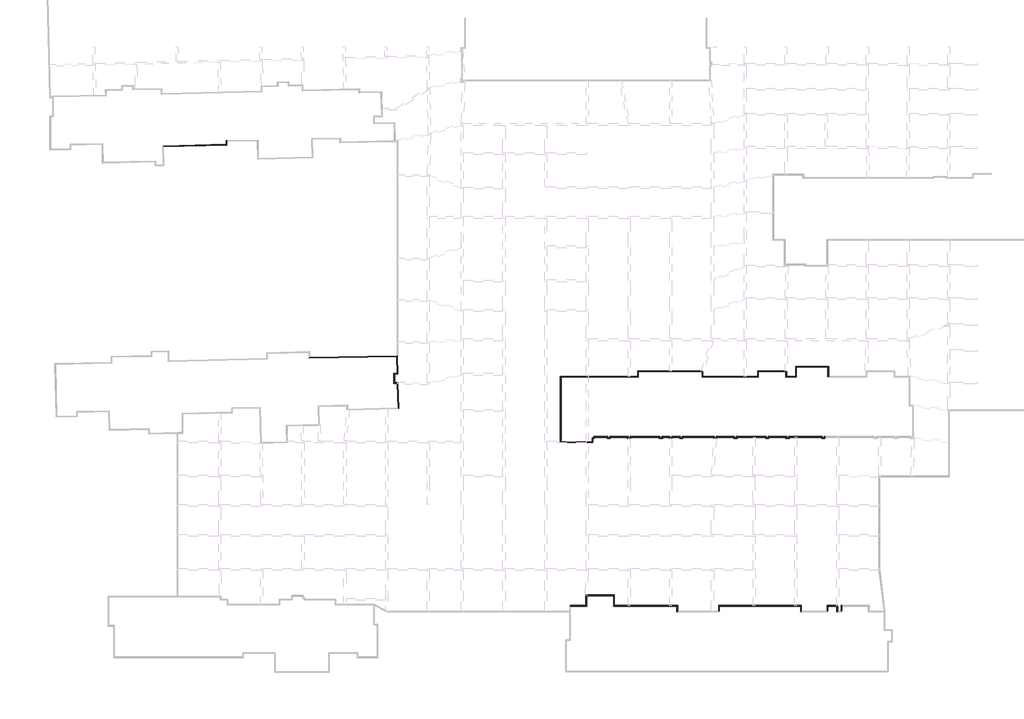
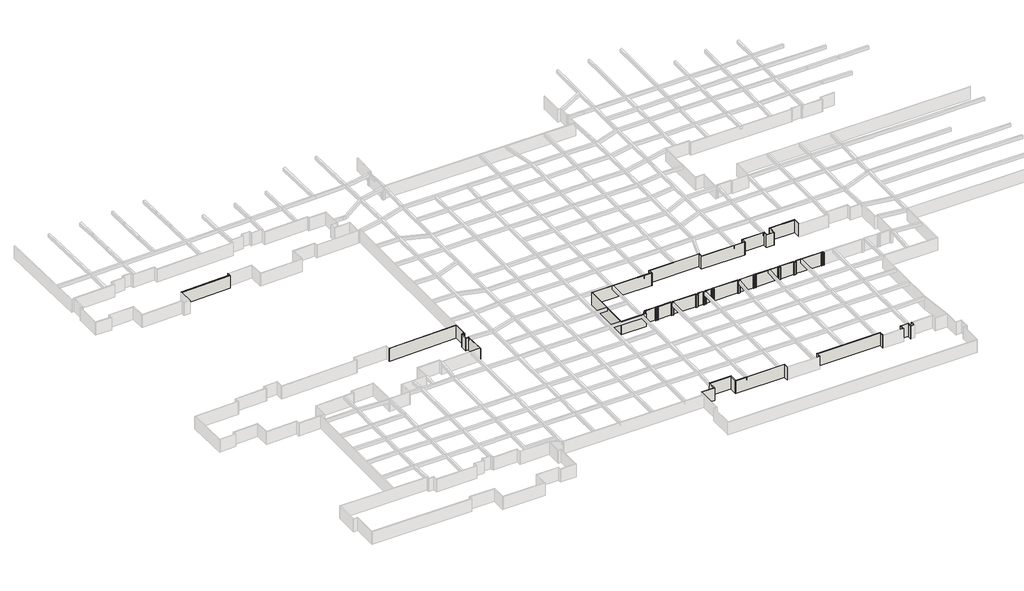
# One storey, part 3 of 20: 78 walls.
"""IFC4 building model written with IfcOpenShell, lengths in millimetres."""

from ifc_helpers import new_model, si_unit, origin, origin_with_axes, place, context, project, spatial, polyline, outline, extrude, faceted_brep, element, save

model = new_model("IFC4")

# Units and contexts
model_context = context("Model", 3, world=origin())
ifc_project = project(units=[si_unit("LENGTHUNIT", "METRE", prefix="MILLI")], contexts=[model_context])

# Site, building, storey
site = spatial("IfcSite", under=ifc_project)
building = spatial("IfcBuilding", under=site)
storey = spatial("IfcBuildingStorey", under=building, Name="户型图", Elevation=0.0)

# Walls
placement = place(None, origin())
element("IfcWall", 1, ObjectType="所有墙体", at=placement, inside=storey, context=model_context, shape_type="Brep", body=[
    faceted_brep([(-2724.8650084, 89257.8239839, 0.0), (9470.1632227, 89551.8005582, 0.0), (9470.1632227, 89551.8005582, 3300.0), (-2724.8650084, 89257.8239839, 3300.0), (-2727.75692, 89377.7891324, 0.0), (-2727.75692, 89377.7891324, 3300.0), (9350.1632227, 89668.9426681, 3300.0), (9470.1632227, 89671.8354198, 3300.0), (9470.1632227, 89671.8354198, 0.0), (9350.1632227, 89668.9426681, 0.0)], [[[0, 1, 2, 3]], [[4, 5, 6, 7, 8, 9]], [[1, 0, 4, 9, 8]], [[3, 2, 7, 6, 5]], [[0, 3, 5, 4]], [[2, 1, 8, 7]]]),
])
element("IfcWall", 2, ObjectType="所有墙体", at=placement, inside=storey, context=model_context, shape_type="Brep", body=[
    faceted_brep([(9470.1632227, 89671.8354198, 0.0), (9470.1632227, 90251.8005582, 0.0), (9470.1632227, 90371.8354198, 0.0), (9470.1632227, 90371.8354198, 3300.0), (9470.1632227, 90251.8005582, 3300.0), (9470.1632227, 89671.8354198, 3300.0), (9350.1632227, 89668.9426681, 0.0), (9350.1632227, 89668.9426681, 3300.0), (9350.1632227, 90368.9426681, 3300.0), (9350.1632227, 90368.9426681, 0.0)], [[[0, 1, 2, 3, 4, 5]], [[6, 7, 8, 9]], [[2, 1, 0, 6, 9]], [[5, 4, 3, 8, 7]], [[0, 5, 7, 6]], [[3, 2, 9, 8]]]),
])
element("IfcWall", 3, ObjectType="所有墙体", at=placement, inside=storey, context=model_context, shape_type="Brep", body=[
    faceted_brep([(42190.0, 49087.0906084, 0.0), (25412.5739519, 48794.2395474, 0.0), (25292.5739519, 48792.1449396, 0.0), (25292.5739519, 48792.1449396, 3300.0), (25412.5739519, 48794.2395474, 3300.0), (42190.0, 49087.0906084, 3300.0), (42190.0, 48967.072329, 0.0), (42190.0, 48967.072329, 3300.0), (42078.6480995, 48965.1286744, 3300.0), (25292.5739519, 48672.1266602, 3300.0), (25292.5739519, 48672.1266602, 0.0), (42078.6480995, 48965.1286744, 0.0)], [[[0, 1, 2, 3, 4, 5]], [[6, 7, 8, 9, 10, 11]], [[2, 1, 0, 6, 11, 10]], [[5, 4, 3, 9, 8, 7]], [[0, 5, 7, 6]], [[3, 2, 10, 9]]]),
])
element("IfcWall", 4, ObjectType="所有墙体", at=placement, inside=storey, context=model_context, shape_type="Brep", body=[
    faceted_brep([(75347.25326, 1046.0, 0.0), (78482.0, 1046.0, 0.0), (78482.0, 1046.0, 3300.0), (75347.25326, 1046.0, 3300.0), (75347.25326, 1166.0, 0.0), (75347.25326, 1166.0, 3300.0), (78362.0, 1166.0, 3300.0), (78482.0, 1166.0, 3300.0), (78482.0, 1166.0, 0.0), (78362.0, 1166.0, 0.0)], [[[0, 1, 2, 3]], [[4, 5, 6, 7, 8, 9]], [[1, 0, 4, 9, 8]], [[3, 2, 7, 6, 5]], [[0, 3, 5, 4]], [[2, 1, 8, 7]]]),
])
element("IfcWall", 5, ObjectType="所有墙体", at=placement, inside=storey, context=model_context, shape_type="Brep", body=[
    faceted_brep([(78482.0, 1166.0, 0.0), (78482.0, 3045.0, 0.0), (78482.0, 3165.0, 0.0), (78482.0, 3165.0, 3300.0), (78482.0, 3045.0, 3300.0), (78482.0, 1166.0, 3300.0), (78362.0, 1166.0, 0.0), (78362.0, 1166.0, 3300.0), (78362.0, 3165.0, 3300.0), (78362.0, 3165.0, 0.0)], [[[0, 1, 2, 3, 4, 5]], [[6, 7, 8, 9]], [[2, 1, 0, 6, 9]], [[5, 4, 3, 8, 7]], [[0, 5, 7, 6]], [[3, 2, 9, 8]]]),
])
element("IfcWall", 6, ObjectType="所有墙体", at=placement, inside=storey, context=model_context, shape_type="Brep", body=[
    faceted_brep([(78482.0, 3045.0, 0.0), (83662.0, 3045.0, 0.0), (83782.0, 3045.0, 0.0), (83782.0, 3045.0, 3300.0), (83662.0, 3045.0, 3300.0), (78482.0, 3045.0, 3300.0), (78482.0, 3165.0, 0.0), (78482.0, 3165.0, 3300.0), (83782.0, 3165.0, 3300.0), (83782.0, 3165.0, 0.0)], [[[0, 1, 2, 3, 4, 5]], [[6, 7, 8, 9]], [[2, 1, 0, 6, 9]], [[5, 4, 3, 8, 7]], [[0, 5, 7, 6]], [[3, 2, 9, 8]]]),
])
element("IfcWall", 7, ObjectType="所有墙体", at=placement, inside=storey, context=model_context, shape_type="Brep", body=[
    faceted_brep([(83662.0, 3045.0, 0.0), (83662.0, 1046.0, 0.0), (83662.0, 1046.0, 3300.0), (83662.0, 3045.0, 3300.0), (83782.0, 3045.0, 0.0), (83782.0, 3045.0, 3300.0), (83782.0, 1166.0, 3300.0), (83782.0, 1046.0, 3300.0), (83782.0, 1046.0, 0.0), (83782.0, 1166.0, 0.0)], [[[0, 1, 2, 3]], [[4, 5, 6, 7, 8, 9]], [[1, 0, 4, 9, 8]], [[3, 2, 7, 6, 5]], [[0, 3, 5, 4]], [[2, 1, 8, 7]]]),
])
element("IfcWall", 8, ObjectType="所有墙体", at=placement, inside=storey, context=model_context, shape_type="Brep", body=[
    faceted_brep([(83782.0, 1046.0, 0.0), (95812.0, 1046.0, 0.0), (95932.0, 1046.0, 0.0), (95932.0, 1046.0, 3300.0), (95812.0, 1046.0, 3300.0), (83782.0, 1046.0, 3300.0), (83782.0, 1166.0, 0.0), (83782.0, 1166.0, 3300.0), (95932.0, 1166.0, 3300.0), (95932.0, 1166.0, 0.0)], [[[0, 1, 2, 3, 4, 5]], [[6, 7, 8, 9]], [[2, 1, 0, 6, 9]], [[5, 4, 3, 8, 7]], [[0, 5, 7, 6]], [[3, 2, 9, 8]]]),
])
element("IfcWall", 9, ObjectType="所有墙体", at=placement, inside=storey, context=model_context, shape_type="Brep", body=[
    faceted_brep([(95812.0, 1046.0, 0.0), (95812.0, -63.5203758, 0.0), (95812.0, -63.5203758, 3300.0), (95812.0, 1046.0, 3300.0), (95932.0, 1046.0, 0.0), (95932.0, 1046.0, 3300.0), (95932.0, 56.4796242, 3300.0), (95932.0, -63.5203758, 3300.0), (95932.0, -63.5203758, 0.0), (95932.0, 56.4796242, 0.0)], [[[0, 1, 2, 3]], [[4, 5, 6, 7, 8, 9]], [[1, 0, 4, 9, 8]], [[3, 2, 7, 6, 5]], [[0, 3, 5, 4]], [[2, 1, 8, 7]]]),
])
element("IfcWall", 10, ObjectType="所有墙体", at=placement, inside=storey, context=model_context, shape_type="Brep", body=[
    faceted_brep([(103982.0, 56.4796242, 0.0), (103982.0, 1046.0, 0.0), (103982.0, 1166.0, 0.0), (103982.0, 1166.0, 3300.0), (103982.0, 1046.0, 3300.0), (103982.0, 56.4796242, 3300.0), (103862.0, 56.4796242, 0.0), (103862.0, 56.4796242, 3300.0), (103862.0, 1166.0, 3300.0), (103862.0, 1166.0, 0.0)], [[[0, 1, 2, 3, 4, 5]], [[6, 7, 8, 9]], [[2, 1, 0, 6, 9]], [[5, 4, 3, 8, 7]], [[0, 5, 7, 6]], [[3, 2, 9, 8]]]),
])
element("IfcWall", 11, ObjectType="所有墙体", at=placement, inside=storey, context=model_context, shape_type="Brep", body=[
    faceted_brep([(103982.0, 1046.0, 0.0), (119562.0, 1046.0, 0.0), (119682.0, 1046.0, 0.0), (119682.0, 1046.0, 3300.0), (119562.0, 1046.0, 3300.0), (103982.0, 1046.0, 3300.0), (103982.0, 1166.0, 0.0), (103982.0, 1166.0, 3300.0), (119682.0, 1166.0, 3300.0), (119682.0, 1166.0, 0.0)], [[[0, 1, 2, 3, 4, 5]], [[6, 7, 8, 9]], [[2, 1, 0, 6, 9]], [[5, 4, 3, 8, 7]], [[0, 5, 7, 6]], [[3, 2, 9, 8]]]),
])
element("IfcWall", 12, ObjectType="所有墙体", at=placement, inside=storey, context=model_context, shape_type="Brep", body=[
    faceted_brep([(119562.0, 1046.0, 0.0), (119562.0, -63.5203758, 0.0), (119562.0, -63.5203758, 3300.0), (119562.0, 1046.0, 3300.0), (119682.0, 1046.0, 0.0), (119682.0, 1046.0, 3300.0), (119682.0, 56.4796242, 3300.0), (119682.0, -63.5203758, 3300.0), (119682.0, -63.5203758, 0.0), (119682.0, 56.4796242, 0.0)], [[[0, 1, 2, 3]], [[4, 5, 6, 7, 8, 9]], [[1, 0, 4, 9, 8]], [[3, 2, 7, 6, 5]], [[0, 3, 5, 4]], [[2, 1, 8, 7]]]),
])
element("IfcWall", 13, ObjectType="所有墙体", at=placement, inside=storey, context=model_context, shape_type="Brep", body=[
    faceted_brep([(124732.0, 56.4796242, 0.0), (124732.0, 1046.0, 0.0), (124732.0, 1166.0, 0.0), (124732.0, 1166.0, 3300.0), (124732.0, 1046.0, 3300.0), (124732.0, 56.4796242, 3300.0), (124612.0, 56.4796242, 0.0), (124612.0, 56.4796242, 3300.0), (124612.0, 1166.0, 3300.0), (124612.0, 1166.0, 0.0)], [[[0, 1, 2, 3, 4, 5]], [[6, 7, 8, 9]], [[2, 1, 0, 6, 9]], [[5, 4, 3, 8, 7]], [[0, 5, 7, 6]], [[3, 2, 9, 8]]]),
])
element("IfcWall", 14, ObjectType="所有墙体", at=placement, inside=storey, context=model_context, shape_type="Brep", body=[
    faceted_brep([(124732.0, 1046.0, 0.0), (126512.0, 1046.0, 0.0), (126632.0, 1046.0, 0.0), (126632.0, 1046.0, 3300.0), (126512.0, 1046.0, 3300.0), (124732.0, 1046.0, 3300.0), (124732.0, 1166.0, 0.0), (124732.0, 1166.0, 3300.0), (126632.0, 1166.0, 3300.0), (126632.0, 1166.0, 0.0)], [[[0, 1, 2, 3, 4, 5]], [[6, 7, 8, 9]], [[2, 1, 0, 6, 9]], [[5, 4, 3, 8, 7]], [[0, 5, 7, 6]], [[3, 2, 9, 8]]]),
])
element("IfcWall", 15, ObjectType="所有墙体", at=placement, inside=storey, context=model_context, shape_type="Brep", body=[
    faceted_brep([(126512.0, 1046.0, 0.0), (126512.0, -63.5203758, 0.0), (126512.0, -63.5203758, 3300.0), (126512.0, 1046.0, 3300.0), (126632.0, 1046.0, 0.0), (126632.0, 1046.0, 3300.0), (126632.0, 56.4796242, 3300.0), (126632.0, -63.5203758, 3300.0), (126632.0, -63.5203758, 0.0), (126632.0, 56.4796242, 0.0)], [[[0, 1, 2, 3]], [[4, 5, 6, 7, 8, 9]], [[1, 0, 4, 9, 8]], [[3, 2, 7, 6, 5]], [[0, 3, 5, 4]], [[2, 1, 8, 7]]]),
])
element("IfcWall", 16, ObjectType="所有墙体", at=placement, inside=storey, context=model_context, shape_type="Brep", body=[
    faceted_brep([(127432.0, 56.4796242, 0.0), (127432.0, 1046.0, 0.0), (127432.0, 1166.0, 0.0), (127432.0, 1166.0, 3300.0), (127432.0, 1046.0, 3300.0), (127432.0, 56.4796242, 3300.0), (127312.0, 56.4796242, 0.0), (127312.0, 56.4796242, 3300.0), (127312.0, 1166.0, 3300.0), (127312.0, 1166.0, 0.0)], [[[0, 1, 2, 3, 4, 5]], [[6, 7, 8, 9]], [[2, 1, 0, 6, 9]], [[5, 4, 3, 8, 7]], [[0, 5, 7, 6]], [[3, 2, 9, 8]]]),
])
element("IfcWall", 17, ObjectType="所有墙体", at=placement, inside=storey, context=model_context, shape_type="Brep", body=[
    faceted_brep([(73484.0, 45158.2500378, 0.0), (73484.0, 32431.88725, 0.0), (73484.0, 32431.88725, 3300.0), (73484.0, 45158.2500378, 3300.0), (73604.0, 45158.2500378, 0.0), (73604.0, 45158.2500378, 3300.0), (73604.0, 45038.2500378, 3300.0), (73604.0, 32551.88725, 3300.0), (73604.0, 32431.88725, 3300.0), (73604.0, 32431.88725, 0.0), (73604.0, 32551.88725, 0.0), (73604.0, 45038.2500378, 0.0)], [[[0, 1, 2, 3]], [[4, 5, 6, 7, 8, 9, 10, 11]], [[1, 0, 4, 11, 10, 9]], [[3, 2, 8, 7, 6, 5]], [[2, 1, 9, 8]], [[0, 3, 5, 4]]]),
])
element("IfcWall", 18, ObjectType="所有墙体", at=placement, inside=storey, context=model_context, shape_type="Brep", body=[
    faceted_brep([(73604.0, 32431.88725, 0.0), (79654.0, 32431.88725, 0.0), (79654.0, 32431.88725, 3300.0), (73604.0, 32431.88725, 3300.0), (73604.0, 32551.88725, 0.0), (73604.0, 32551.88725, 3300.0), (79534.0, 32551.88725, 3300.0), (79654.0, 32551.88725, 3300.0), (79654.0, 32551.88725, 0.0), (79534.0, 32551.88725, 0.0)], [[[0, 1, 2, 3]], [[4, 5, 6, 7, 8, 9]], [[1, 0, 4, 9, 8]], [[3, 2, 7, 6, 5]], [[0, 3, 5, 4]], [[2, 1, 8, 7]]]),
])
element("IfcWall", 19, ObjectType="所有墙体", at=placement, inside=storey, context=model_context, shape_type="SweptSolid", body=[
    extrude(outline(polyline([(79654.0, 33197.0), (79654.0, 32551.88725), (79534.0, 32551.88725), (79534.0, 33197.0), (79654.0, 33197.0)])), origin_with_axes(), (0.0, 0.0, 1.0), 3300.0),
])
element("IfcWall", 20, ObjectType="所有墙体", at=placement, inside=storey, context=model_context, shape_type="Brep", body=[
    faceted_brep([(79534.0, 33197.0, 0.0), (79654.0, 33197.0, 0.0), (79954.0, 33197.0, 0.0), (79954.0, 33197.0, 3300.0), (79654.0, 33197.0, 3300.0), (79534.0, 33197.0, 3300.0), (79534.0, 33317.0, 0.0), (79534.0, 33317.0, 3300.0), (79834.0, 33317.0, 3300.0), (79954.0, 33317.0, 3300.0), (79954.0, 33317.0, 0.0), (79834.0, 33317.0, 0.0)], [[[0, 1, 2, 3, 4, 5]], [[6, 7, 8, 9, 10, 11]], [[2, 1, 0, 6, 11, 10]], [[5, 4, 3, 9, 8, 7]], [[0, 5, 7, 6]], [[3, 2, 10, 9]]]),
])
element("IfcWall", 21, ObjectType="所有墙体", at=placement, inside=storey, context=model_context, shape_type="Brep", body=[
    faceted_brep([(79954.0, 33317.0, 0.0), (79954.0, 33447.0, 0.0), (79954.0, 33567.0, 0.0), (79954.0, 33567.0, 3300.0), (79954.0, 33447.0, 3300.0), (79954.0, 33317.0, 3300.0), (79834.0, 33317.0, 0.0), (79834.0, 33317.0, 3300.0), (79834.0, 33567.0, 3300.0), (79834.0, 33567.0, 0.0)], [[[0, 1, 2, 3, 4, 5]], [[6, 7, 8, 9]], [[2, 1, 0, 6, 9]], [[5, 4, 3, 8, 7]], [[0, 5, 7, 6]], [[3, 2, 9, 8]]]),
])
element("IfcWall", 22, ObjectType="所有墙体", at=placement, inside=storey, context=model_context, shape_type="SweptSolid", body=[
    extrude(outline(polyline([(82434.0, 33447.0), (79954.0, 33447.0), (79954.0, 33567.0), (82434.0, 33567.0), (82434.0, 33447.0)])), origin_with_axes(), (0.0, 0.0, 1.0), 3300.0),
])
element("IfcWall", 23, ObjectType="所有墙体", at=placement, inside=storey, context=model_context, shape_type="Brep", body=[
    faceted_brep([(82434.0, 33567.0, 0.0), (82434.0, 33447.0, 0.0), (82434.0, 33197.0, 0.0), (82434.0, 33197.0, 3300.0), (82434.0, 33447.0, 3300.0), (82434.0, 33567.0, 3300.0), (82554.0, 33567.0, 0.0), (82554.0, 33567.0, 3300.0), (82554.0, 33317.0, 3300.0), (82554.0, 33197.0, 3300.0), (82554.0, 33197.0, 0.0), (82554.0, 33317.0, 0.0)], [[[0, 1, 2, 3, 4, 5]], [[6, 7, 8, 9, 10, 11]], [[2, 1, 0, 6, 11, 10]], [[5, 4, 3, 9, 8, 7]], [[0, 5, 7, 6]], [[3, 2, 10, 9]]]),
])
element("IfcWall", 24, ObjectType="所有墙体", at=placement, inside=storey, context=model_context, shape_type="SweptSolid", body=[
    extrude(outline(polyline([(82934.0, 33197.0), (82554.0, 33197.0), (82554.0, 33317.0), (82934.0, 33317.0), (82934.0, 33197.0)])), origin_with_axes(), (0.0, 0.0, 1.0), 3300.0),
])
element("IfcWall", 25, ObjectType="所有墙体", at=placement, inside=storey, context=model_context, shape_type="Brep", body=[
    faceted_brep([(83054.0, 33197.0, 0.0), (83054.0, 33447.0, 0.0), (83054.0, 33567.0, 0.0), (83054.0, 33567.0, 3300.0), (83054.0, 33447.0, 3300.0), (83054.0, 33197.0, 3300.0), (82934.0, 33197.0, 0.0), (82934.0, 33197.0, 3300.0), (82934.0, 33317.0, 3300.0), (82934.0, 33567.0, 3300.0), (82934.0, 33567.0, 0.0), (82934.0, 33317.0, 0.0)], [[[0, 1, 2, 3, 4, 5]], [[6, 7, 8, 9, 10, 11]], [[2, 1, 0, 6, 11, 10]], [[5, 4, 3, 9, 8, 7]], [[0, 5, 7, 6]], [[3, 2, 10, 9]]]),
])
element("IfcWall", 26, ObjectType="所有墙体", at=placement, inside=storey, context=model_context, shape_type="SweptSolid", body=[
    extrude(outline(polyline([(86334.0, 33447.0), (83054.0, 33447.0), (83054.0, 33567.0), (86334.0, 33567.0), (86334.0, 33447.0)])), origin_with_axes(), (0.0, 0.0, 1.0), 3300.0),
])
element("IfcWall", 27, ObjectType="所有墙体", at=placement, inside=storey, context=model_context, shape_type="Brep", body=[
    faceted_brep([(86334.0, 33567.0, 0.0), (86334.0, 33447.0, 0.0), (86334.0, 33197.0, 0.0), (86334.0, 33197.0, 3300.0), (86334.0, 33447.0, 3300.0), (86334.0, 33567.0, 3300.0), (86454.0, 33567.0, 0.0), (86454.0, 33567.0, 3300.0), (86454.0, 33317.0, 3300.0), (86454.0, 33197.0, 3300.0), (86454.0, 33197.0, 0.0), (86454.0, 33317.0, 0.0)], [[[0, 1, 2, 3, 4, 5]], [[6, 7, 8, 9, 10, 11]], [[2, 1, 0, 6, 11, 10]], [[5, 4, 3, 9, 8, 7]], [[0, 5, 7, 6]], [[3, 2, 10, 9]]]),
])
element("IfcWall", 28, ObjectType="所有墙体", at=placement, inside=storey, context=model_context, shape_type="SweptSolid", body=[
    extrude(outline(polyline([(86834.0, 33197.0), (86454.0, 33197.0), (86454.0, 33317.0), (86834.0, 33317.0), (86834.0, 33197.0)])), origin_with_axes(), (0.0, 0.0, 1.0), 3300.0),
])
element("IfcWall", 29, ObjectType="所有墙体", at=placement, inside=storey, context=model_context, shape_type="Brep", body=[
    faceted_brep([(86954.0, 33197.0, 0.0), (86954.0, 33447.0, 0.0), (86954.0, 33567.0, 0.0), (86954.0, 33567.0, 3300.0), (86954.0, 33447.0, 3300.0), (86954.0, 33197.0, 3300.0), (86834.0, 33197.0, 0.0), (86834.0, 33197.0, 3300.0), (86834.0, 33317.0, 3300.0), (86834.0, 33567.0, 3300.0), (86834.0, 33567.0, 0.0), (86834.0, 33317.0, 0.0)], [[[0, 1, 2, 3, 4, 5]], [[6, 7, 8, 9, 10, 11]], [[2, 1, 0, 6, 11, 10]], [[5, 4, 3, 9, 8, 7]], [[0, 5, 7, 6]], [[3, 2, 10, 9]]]),
])
element("IfcWall", 30, ObjectType="所有墙体", at=placement, inside=storey, context=model_context, shape_type="SweptSolid", body=[
    extrude(outline(polyline([(92434.0, 33447.0), (86954.0, 33447.0), (86954.0, 33567.0), (92434.0, 33567.0), (92434.0, 33447.0)])), origin_with_axes(), (0.0, 0.0, 1.0), 3300.0),
])
element("IfcWall", 31, ObjectType="所有墙体", at=placement, inside=storey, context=model_context, shape_type="Brep", body=[
    faceted_brep([(92434.0, 33567.0, 0.0), (92434.0, 33447.0, 0.0), (92434.0, 33197.0, 0.0), (92434.0, 33197.0, 3300.0), (92434.0, 33447.0, 3300.0), (92434.0, 33567.0, 3300.0), (92554.0, 33567.0, 0.0), (92554.0, 33567.0, 3300.0), (92554.0, 33317.0, 3300.0), (92554.0, 33197.0, 3300.0), (92554.0, 33197.0, 0.0), (92554.0, 33317.0, 0.0)], [[[0, 1, 2, 3, 4, 5]], [[6, 7, 8, 9, 10, 11]], [[2, 1, 0, 6, 11, 10]], [[5, 4, 3, 9, 8, 7]], [[0, 5, 7, 6]], [[3, 2, 10, 9]]]),
])
element("IfcWall", 32, ObjectType="所有墙体", at=placement, inside=storey, context=model_context, shape_type="SweptSolid", body=[
    extrude(outline(polyline([(92934.0, 33197.0), (92554.0, 33197.0), (92554.0, 33317.0), (92934.0, 33317.0), (92934.0, 33197.0)])), origin_with_axes(), (0.0, 0.0, 1.0), 3300.0),
])
element("IfcWall", 33, ObjectType="所有墙体", at=placement, inside=storey, context=model_context, shape_type="Brep", body=[
    faceted_brep([(93054.0, 33197.0, 0.0), (93054.0, 33447.0, 0.0), (93054.0, 33567.0, 0.0), (93054.0, 33567.0, 3300.0), (93054.0, 33447.0, 3300.0), (93054.0, 33197.0, 3300.0), (92934.0, 33197.0, 0.0), (92934.0, 33197.0, 3300.0), (92934.0, 33317.0, 3300.0), (92934.0, 33567.0, 3300.0), (92934.0, 33567.0, 0.0), (92934.0, 33317.0, 0.0)], [[[0, 1, 2, 3, 4, 5]], [[6, 7, 8, 9, 10, 11]], [[2, 1, 0, 6, 11, 10]], [[5, 4, 3, 9, 8, 7]], [[0, 5, 7, 6]], [[3, 2, 10, 9]]]),
])
element("IfcWall", 34, ObjectType="所有墙体", at=placement, inside=storey, context=model_context, shape_type="SweptSolid", body=[
    extrude(outline(polyline([(94335.0, 33447.0), (93054.0, 33447.0), (93054.0, 33567.0), (94335.0, 33567.0), (94335.0, 33447.0)])), origin_with_axes(), (0.0, 0.0, 1.0), 3300.0),
])
element("IfcWall", 35, ObjectType="所有墙体", at=placement, inside=storey, context=model_context, shape_type="Brep", body=[
    faceted_brep([(94335.0, 33567.0, 0.0), (94335.0, 33447.0, 0.0), (94335.0, 33197.0, 0.0), (94335.0, 33197.0, 3300.0), (94335.0, 33447.0, 3300.0), (94335.0, 33567.0, 3300.0), (94455.0, 33567.0, 0.0), (94455.0, 33567.0, 3300.0), (94455.0, 33317.0, 3300.0), (94455.0, 33197.0, 3300.0), (94455.0, 33197.0, 0.0), (94455.0, 33317.0, 0.0)], [[[0, 1, 2, 3, 4, 5]], [[6, 7, 8, 9, 10, 11]], [[2, 1, 0, 6, 11, 10]], [[5, 4, 3, 9, 8, 7]], [[0, 5, 7, 6]], [[3, 2, 10, 9]]]),
])
element("IfcWall", 36, ObjectType="所有墙体", at=placement, inside=storey, context=model_context, shape_type="SweptSolid", body=[
    extrude(outline(polyline([(94835.0, 33197.0), (94455.0, 33197.0), (94455.0, 33317.0), (94835.0, 33317.0), (94835.0, 33197.0)])), origin_with_axes(), (0.0, 0.0, 1.0), 3300.0),
])
element("IfcWall", 37, ObjectType="所有墙体", at=placement, inside=storey, context=model_context, shape_type="Brep", body=[
    faceted_brep([(94955.0, 33197.0, 0.0), (94955.0, 33447.0, 0.0), (94955.0, 33567.0, 0.0), (94955.0, 33567.0, 3300.0), (94955.0, 33447.0, 3300.0), (94955.0, 33197.0, 3300.0), (94835.0, 33197.0, 0.0), (94835.0, 33197.0, 3300.0), (94835.0, 33317.0, 3300.0), (94835.0, 33567.0, 3300.0), (94835.0, 33567.0, 0.0), (94835.0, 33317.0, 0.0)], [[[0, 1, 2, 3, 4, 5]], [[6, 7, 8, 9, 10, 11]], [[2, 1, 0, 6, 11, 10]], [[5, 4, 3, 9, 8, 7]], [[0, 5, 7, 6]], [[3, 2, 10, 9]]]),
])
element("IfcWall", 38, ObjectType="所有墙体", at=placement, inside=storey, context=model_context, shape_type="SweptSolid", body=[
    extrude(outline(polyline([(96334.0, 33447.0), (94955.0, 33447.0), (94955.0, 33567.0), (96334.0, 33567.0), (96334.0, 33447.0)])), origin_with_axes(), (0.0, 0.0, 1.0), 3300.0),
])
element("IfcWall", 39, ObjectType="所有墙体", at=placement, inside=storey, context=model_context, shape_type="Brep", body=[
    faceted_brep([(96334.0, 33567.0, 0.0), (96334.0, 33447.0, 0.0), (96334.0, 33197.0, 0.0), (96334.0, 33197.0, 3300.0), (96334.0, 33447.0, 3300.0), (96334.0, 33567.0, 3300.0), (96454.0, 33567.0, 0.0), (96454.0, 33567.0, 3300.0), (96454.0, 33317.0, 3300.0), (96454.0, 33197.0, 3300.0), (96454.0, 33197.0, 0.0), (96454.0, 33317.0, 0.0)], [[[0, 1, 2, 3, 4, 5]], [[6, 7, 8, 9, 10, 11]], [[2, 1, 0, 6, 11, 10]], [[5, 4, 3, 9, 8, 7]], [[0, 5, 7, 6]], [[3, 2, 10, 9]]]),
])
element("IfcWall", 40, ObjectType="所有墙体", at=placement, inside=storey, context=model_context, shape_type="SweptSolid", body=[
    extrude(outline(polyline([(96834.0, 33197.0), (96454.0, 33197.0), (96454.0, 33317.0), (96834.0, 33317.0), (96834.0, 33197.0)])), origin_with_axes(), (0.0, 0.0, 1.0), 3300.0),
])
element("IfcWall", 41, ObjectType="所有墙体", at=placement, inside=storey, context=model_context, shape_type="Brep", body=[
    faceted_brep([(96954.0, 33197.0, 0.0), (96954.0, 33447.0, 0.0), (96954.0, 33567.0, 0.0), (96954.0, 33567.0, 3300.0), (96954.0, 33447.0, 3300.0), (96954.0, 33197.0, 3300.0), (96834.0, 33197.0, 0.0), (96834.0, 33197.0, 3300.0), (96834.0, 33317.0, 3300.0), (96834.0, 33567.0, 3300.0), (96834.0, 33567.0, 0.0), (96834.0, 33317.0, 0.0)], [[[0, 1, 2, 3, 4, 5]], [[6, 7, 8, 9, 10, 11]], [[2, 1, 0, 6, 11, 10]], [[5, 4, 3, 9, 8, 7]], [[0, 5, 7, 6]], [[3, 2, 10, 9]]]),
])
element("IfcWall", 42, ObjectType="所有墙体", at=placement, inside=storey, context=model_context, shape_type="SweptSolid", body=[
    extrude(outline(polyline([(102834.0, 33447.0), (96954.0, 33447.0), (96954.0, 33567.0), (102834.0, 33567.0), (102834.0, 33447.0)])), origin_with_axes(), (0.0, 0.0, 1.0), 3300.0),
])
element("IfcWall", 43, ObjectType="所有墙体", at=placement, inside=storey, context=model_context, shape_type="Brep", body=[
    faceted_brep([(102834.0, 33567.0, 0.0), (102834.0, 33447.0, 0.0), (102834.0, 33197.0, 0.0), (102834.0, 33197.0, 3300.0), (102834.0, 33447.0, 3300.0), (102834.0, 33567.0, 3300.0), (102954.0, 33567.0, 0.0), (102954.0, 33567.0, 3300.0), (102954.0, 33317.0, 3300.0), (102954.0, 33197.0, 3300.0), (102954.0, 33197.0, 0.0), (102954.0, 33317.0, 0.0)], [[[0, 1, 2, 3, 4, 5]], [[6, 7, 8, 9, 10, 11]], [[2, 1, 0, 6, 11, 10]], [[5, 4, 3, 9, 8, 7]], [[0, 5, 7, 6]], [[3, 2, 10, 9]]]),
])
element("IfcWall", 44, ObjectType="所有墙体", at=placement, inside=storey, context=model_context, shape_type="SweptSolid", body=[
    extrude(outline(polyline([(103334.0, 33197.0), (102954.0, 33197.0), (102954.0, 33317.0), (103334.0, 33317.0), (103334.0, 33197.0)])), origin_with_axes(), (0.0, 0.0, 1.0), 3300.0),
])
element("IfcWall", 45, ObjectType="所有墙体", at=placement, inside=storey, context=model_context, shape_type="Brep", body=[
    faceted_brep([(103454.0, 33197.0, 0.0), (103454.0, 33447.0, 0.0), (103454.0, 33567.0, 0.0), (103454.0, 33567.0, 3300.0), (103454.0, 33447.0, 3300.0), (103454.0, 33197.0, 3300.0), (103334.0, 33197.0, 0.0), (103334.0, 33197.0, 3300.0), (103334.0, 33317.0, 3300.0), (103334.0, 33567.0, 3300.0), (103334.0, 33567.0, 0.0), (103334.0, 33317.0, 0.0)], [[[0, 1, 2, 3, 4, 5]], [[6, 7, 8, 9, 10, 11]], [[2, 1, 0, 6, 11, 10]], [[5, 4, 3, 9, 8, 7]], [[0, 5, 7, 6]], [[3, 2, 10, 9]]]),
])
element("IfcWall", 46, ObjectType="所有墙体", at=placement, inside=storey, context=model_context, shape_type="SweptSolid", body=[
    extrude(outline(polyline([(106734.0, 33447.0), (103454.0, 33447.0), (103454.0, 33567.0), (106734.0, 33567.0), (106734.0, 33447.0)])), origin_with_axes(), (0.0, 0.0, 1.0), 3300.0),
])
element("IfcWall", 47, ObjectType="所有墙体", at=placement, inside=storey, context=model_context, shape_type="Brep", body=[
    faceted_brep([(106734.0, 33567.0, 0.0), (106734.0, 33447.0, 0.0), (106734.0, 33197.0, 0.0), (106734.0, 33197.0, 3300.0), (106734.0, 33447.0, 3300.0), (106734.0, 33567.0, 3300.0), (106854.0, 33567.0, 0.0), (106854.0, 33567.0, 3300.0), (106854.0, 33317.0, 3300.0), (106854.0, 33197.0, 3300.0), (106854.0, 33197.0, 0.0), (106854.0, 33317.0, 0.0)], [[[0, 1, 2, 3, 4, 5]], [[6, 7, 8, 9, 10, 11]], [[2, 1, 0, 6, 11, 10]], [[5, 4, 3, 9, 8, 7]], [[0, 5, 7, 6]], [[3, 2, 10, 9]]]),
])
element("IfcWall", 48, ObjectType="所有墙体", at=placement, inside=storey, context=model_context, shape_type="SweptSolid", body=[
    extrude(outline(polyline([(107234.0, 33197.0), (106854.0, 33197.0), (106854.0, 33317.0), (107234.0, 33317.0), (107234.0, 33197.0)])), origin_with_axes(), (0.0, 0.0, 1.0), 3300.0),
])
element("IfcWall", 49, ObjectType="所有墙体", at=placement, inside=storey, context=model_context, shape_type="Brep", body=[
    faceted_brep([(107354.0, 33197.0, 0.0), (107354.0, 33447.0, 0.0), (107354.0, 33567.0, 0.0), (107354.0, 33567.0, 3300.0), (107354.0, 33447.0, 3300.0), (107354.0, 33197.0, 3300.0), (107234.0, 33197.0, 0.0), (107234.0, 33197.0, 3300.0), (107234.0, 33317.0, 3300.0), (107234.0, 33567.0, 3300.0), (107234.0, 33567.0, 0.0), (107234.0, 33317.0, 0.0)], [[[0, 1, 2, 3, 4, 5]], [[6, 7, 8, 9, 10, 11]], [[2, 1, 0, 6, 11, 10]], [[5, 4, 3, 9, 8, 7]], [[0, 5, 7, 6]], [[3, 2, 10, 9]]]),
])
element("IfcWall", 50, ObjectType="所有墙体", at=placement, inside=storey, context=model_context, shape_type="SweptSolid", body=[
    extrude(outline(polyline([(112834.0, 33447.0), (107354.0, 33447.0), (107354.0, 33567.0), (112834.0, 33567.0), (112834.0, 33447.0)])), origin_with_axes(), (0.0, 0.0, 1.0), 3300.0),
])
element("IfcWall", 51, ObjectType="所有墙体", at=placement, inside=storey, context=model_context, shape_type="Brep", body=[
    faceted_brep([(112834.0, 33567.0, 0.0), (112834.0, 33447.0, 0.0), (112834.0, 33197.0, 0.0), (112834.0, 33197.0, 3300.0), (112834.0, 33447.0, 3300.0), (112834.0, 33567.0, 3300.0), (112954.0, 33567.0, 0.0), (112954.0, 33567.0, 3300.0), (112954.0, 33317.0, 3300.0), (112954.0, 33197.0, 3300.0), (112954.0, 33197.0, 0.0), (112954.0, 33317.0, 0.0)], [[[0, 1, 2, 3, 4, 5]], [[6, 7, 8, 9, 10, 11]], [[2, 1, 0, 6, 11, 10]], [[5, 4, 3, 9, 8, 7]], [[0, 5, 7, 6]], [[3, 2, 10, 9]]]),
])
element("IfcWall", 52, ObjectType="所有墙体", at=placement, inside=storey, context=model_context, shape_type="SweptSolid", body=[
    extrude(outline(polyline([(113334.0, 33197.0), (112954.0, 33197.0), (112954.0, 33317.0), (113334.0, 33317.0), (113334.0, 33197.0)])), origin_with_axes(), (0.0, 0.0, 1.0), 3300.0),
])
element("IfcWall", 53, ObjectType="所有墙体", at=placement, inside=storey, context=model_context, shape_type="Brep", body=[
    faceted_brep([(113454.0, 33197.0, 0.0), (113454.0, 33447.0, 0.0), (113454.0, 33567.0, 0.0), (113454.0, 33567.0, 3300.0), (113454.0, 33447.0, 3300.0), (113454.0, 33197.0, 3300.0), (113334.0, 33197.0, 0.0), (113334.0, 33197.0, 3300.0), (113334.0, 33317.0, 3300.0), (113334.0, 33567.0, 3300.0), (113334.0, 33567.0, 0.0), (113334.0, 33317.0, 0.0)], [[[0, 1, 2, 3, 4, 5]], [[6, 7, 8, 9, 10, 11]], [[2, 1, 0, 6, 11, 10]], [[5, 4, 3, 9, 8, 7]], [[0, 5, 7, 6]], [[3, 2, 10, 9]]]),
])
element("IfcWall", 54, ObjectType="所有墙体", at=placement, inside=storey, context=model_context, shape_type="SweptSolid", body=[
    extrude(outline(polyline([(116734.0, 33447.0), (113454.0, 33447.0), (113454.0, 33567.0), (116734.0, 33567.0), (116734.0, 33447.0)])), origin_with_axes(), (0.0, 0.0, 1.0), 3300.0),
])
element("IfcWall", 55, ObjectType="所有墙体", at=placement, inside=storey, context=model_context, shape_type="Brep", body=[
    faceted_brep([(116734.0, 33567.0, 0.0), (116734.0, 33447.0, 0.0), (116734.0, 33197.0, 0.0), (116734.0, 33197.0, 3300.0), (116734.0, 33447.0, 3300.0), (116734.0, 33567.0, 3300.0), (116854.0, 33567.0, 0.0), (116854.0, 33567.0, 3300.0), (116854.0, 33317.0, 3300.0), (116854.0, 33197.0, 3300.0), (116854.0, 33197.0, 0.0), (116854.0, 33317.0, 0.0)], [[[0, 1, 2, 3, 4, 5]], [[6, 7, 8, 9, 10, 11]], [[2, 1, 0, 6, 11, 10]], [[5, 4, 3, 9, 8, 7]], [[0, 5, 7, 6]], [[3, 2, 10, 9]]]),
])
element("IfcWall", 56, ObjectType="所有墙体", at=placement, inside=storey, context=model_context, shape_type="SweptSolid", body=[
    extrude(outline(polyline([(117234.0, 33197.0), (116854.0, 33197.0), (116854.0, 33317.0), (117234.0, 33317.0), (117234.0, 33197.0)])), origin_with_axes(), (0.0, 0.0, 1.0), 3300.0),
])
element("IfcWall", 57, ObjectType="所有墙体", at=placement, inside=storey, context=model_context, shape_type="Brep", body=[
    faceted_brep([(117354.0, 33197.0, 0.0), (117354.0, 33447.0, 0.0), (117354.0, 33567.0, 0.0), (117354.0, 33567.0, 3300.0), (117354.0, 33447.0, 3300.0), (117354.0, 33197.0, 3300.0), (117234.0, 33197.0, 0.0), (117234.0, 33197.0, 3300.0), (117234.0, 33317.0, 3300.0), (117234.0, 33567.0, 3300.0), (117234.0, 33567.0, 0.0), (117234.0, 33317.0, 0.0)], [[[0, 1, 2, 3, 4, 5]], [[6, 7, 8, 9, 10, 11]], [[2, 1, 0, 6, 11, 10]], [[5, 4, 3, 9, 8, 7]], [[0, 5, 7, 6]], [[3, 2, 10, 9]]]),
])
element("IfcWall", 58, ObjectType="所有墙体", at=placement, inside=storey, context=model_context, shape_type="SweptSolid", body=[
    extrude(outline(polyline([(123584.0, 33447.0), (117354.0, 33447.0), (117354.0, 33567.0), (123584.0, 33567.0), (123584.0, 33447.0)])), origin_with_axes(), (0.0, 0.0, 1.0), 3300.0),
])
element("IfcWall", 59, ObjectType="所有墙体", at=placement, inside=storey, context=model_context, shape_type="Brep", body=[
    faceted_brep([(123584.0, 33567.0, 0.0), (123584.0, 33447.0, 0.0), (123584.0, 33197.0, 0.0), (123584.0, 33197.0, 3300.0), (123584.0, 33447.0, 3300.0), (123584.0, 33567.0, 3300.0), (123704.0, 33567.0, 0.0), (123704.0, 33567.0, 3300.0), (123704.0, 33317.0, 3300.0), (123704.0, 33197.0, 3300.0), (123704.0, 33197.0, 0.0), (123704.0, 33317.0, 0.0)], [[[0, 1, 2, 3, 4, 5]], [[6, 7, 8, 9, 10, 11]], [[2, 1, 0, 6, 11, 10]], [[5, 4, 3, 9, 8, 7]], [[0, 5, 7, 6]], [[3, 2, 10, 9]]]),
])
element("IfcWall", 60, ObjectType="所有墙体", at=placement, inside=storey, context=model_context, shape_type="SweptSolid", body=[
    extrude(outline(polyline([(124084.0, 33197.0), (123704.0, 33197.0), (123704.0, 33317.0), (124084.0, 33317.0), (124084.0, 33197.0)])), origin_with_axes(), (0.0, 0.0, 1.0), 3300.0),
])
element("IfcWall", 61, ObjectType="所有墙体", at=placement, inside=storey, context=model_context, shape_type="Brep", body=[
    faceted_brep([(124204.0, 33197.0, 0.0), (124204.0, 33447.0, 0.0), (124204.0, 33567.0, 0.0), (124204.0, 33567.0, 3300.0), (124204.0, 33447.0, 3300.0), (124204.0, 33197.0, 3300.0), (124084.0, 33197.0, 0.0), (124084.0, 33197.0, 3300.0), (124084.0, 33317.0, 3300.0), (124084.0, 33567.0, 3300.0), (124084.0, 33567.0, 0.0), (124084.0, 33317.0, 0.0)], [[[0, 1, 2, 3, 4, 5]], [[6, 7, 8, 9, 10, 11]], [[2, 1, 0, 6, 11, 10]], [[5, 4, 3, 9, 8, 7]], [[0, 5, 7, 6]], [[3, 2, 10, 9]]]),
])
element("IfcWall", 62, ObjectType="所有墙体", at=placement, inside=storey, context=model_context, shape_type="Brep", body=[
    faceted_brep([(124911.0, 45158.2500378, 0.0), (124911.0, 47018.0, 0.0), (124911.0, 47018.0, 3300.0), (124911.0, 45158.2500378, 3300.0), (124791.0, 45158.2500378, 0.0), (124791.0, 45158.2500378, 3300.0), (124791.0, 46898.0, 3300.0), (124791.0, 47018.0, 3300.0), (124791.0, 47018.0, 0.0), (124791.0, 46898.0, 0.0)], [[[0, 1, 2, 3]], [[4, 5, 6, 7, 8, 9]], [[1, 0, 4, 9, 8]], [[3, 2, 7, 6, 5]], [[0, 3, 5, 4]], [[2, 1, 8, 7]]]),
])
element("IfcWall", 63, ObjectType="所有墙体", at=placement, inside=storey, context=model_context, shape_type="Brep", body=[
    faceted_brep([(124791.0, 47018.0, 0.0), (118584.0, 47018.0, 0.0), (118584.0, 47018.0, 3300.0), (124791.0, 47018.0, 3300.0), (124791.0, 46898.0, 0.0), (124791.0, 46898.0, 3300.0), (118704.0, 46898.0, 3300.0), (118584.0, 46898.0, 3300.0), (118584.0, 46898.0, 0.0), (118704.0, 46898.0, 0.0)], [[[0, 1, 2, 3]], [[4, 5, 6, 7, 8, 9]], [[1, 0, 4, 9, 8]], [[3, 2, 7, 6, 5]], [[0, 3, 5, 4]], [[2, 1, 8, 7]]]),
])
element("IfcWall", 64, ObjectType="所有墙体", at=placement, inside=storey, context=model_context, shape_type="Brep", body=[
    faceted_brep([(118584.0, 46898.0, 0.0), (118584.0, 45158.2500378, 0.0), (118584.0, 45038.2500378, 0.0), (118584.0, 45038.2500378, 3300.0), (118584.0, 45158.2500378, 3300.0), (118584.0, 46898.0, 3300.0), (118704.0, 46898.0, 0.0), (118704.0, 46898.0, 3300.0), (118704.0, 45038.2500378, 3300.0), (118704.0, 45038.2500378, 0.0)], [[[0, 1, 2, 3, 4, 5]], [[6, 7, 8, 9]], [[2, 1, 0, 6, 9]], [[5, 4, 3, 8, 7]], [[0, 5, 7, 6]], [[3, 2, 9, 8]]]),
])
element("IfcWall", 65, ObjectType="所有墙体", at=placement, inside=storey, context=model_context, shape_type="Brep", body=[
    faceted_brep([(118584.0, 45158.2500378, 0.0), (116854.0, 45158.2500378, 0.0), (116734.0, 45158.2500378, 0.0), (116734.0, 45158.2500378, 3300.0), (116854.0, 45158.2500378, 3300.0), (118584.0, 45158.2500378, 3300.0), (118584.0, 45038.2500378, 0.0), (118584.0, 45038.2500378, 3300.0), (116734.0, 45038.2500378, 3300.0), (116734.0, 45038.2500378, 0.0)], [[[0, 1, 2, 3, 4, 5]], [[6, 7, 8, 9]], [[2, 1, 0, 6, 9]], [[5, 4, 3, 8, 7]], [[0, 5, 7, 6]], [[3, 2, 9, 8]]]),
])
element("IfcWall", 66, ObjectType="所有墙体", at=placement, inside=storey, context=model_context, shape_type="Brep", body=[
    faceted_brep([(116854.0, 45158.2500378, 0.0), (116854.0, 46218.0, 0.0), (116854.0, 46218.0, 3300.0), (116854.0, 45158.2500378, 3300.0), (116734.0, 45158.2500378, 0.0), (116734.0, 45158.2500378, 3300.0), (116734.0, 46098.0, 3300.0), (116734.0, 46218.0, 3300.0), (116734.0, 46218.0, 0.0), (116734.0, 46098.0, 0.0)], [[[0, 1, 2, 3]], [[4, 5, 6, 7, 8, 9]], [[1, 0, 4, 9, 8]], [[3, 2, 7, 6, 5]], [[0, 3, 5, 4]], [[2, 1, 8, 7]]]),
])
element("IfcWall", 67, ObjectType="所有墙体", at=placement, inside=storey, context=model_context, shape_type="Brep", body=[
    faceted_brep([(116734.0, 46218.0, 0.0), (111334.0, 46218.0, 0.0), (111334.0, 46218.0, 3300.0), (116734.0, 46218.0, 3300.0), (116734.0, 46098.0, 0.0), (116734.0, 46098.0, 3300.0), (111454.0, 46098.0, 3300.0), (111334.0, 46098.0, 3300.0), (111334.0, 46098.0, 0.0), (111454.0, 46098.0, 0.0)], [[[0, 1, 2, 3]], [[4, 5, 6, 7, 8, 9]], [[1, 0, 4, 9, 8]], [[3, 2, 7, 6, 5]], [[0, 3, 5, 4]], [[2, 1, 8, 7]]]),
])
element("IfcWall", 68, ObjectType="所有墙体", at=placement, inside=storey, context=model_context, shape_type="Brep", body=[
    faceted_brep([(111334.0, 46098.0, 0.0), (111334.0, 45158.2500378, 0.0), (111334.0, 45038.2500378, 0.0), (111334.0, 45038.2500378, 3300.0), (111334.0, 45158.2500378, 3300.0), (111334.0, 46098.0, 3300.0), (111454.0, 46098.0, 0.0), (111454.0, 46098.0, 3300.0), (111454.0, 45038.2500378, 3300.0), (111454.0, 45038.2500378, 0.0)], [[[0, 1, 2, 3, 4, 5]], [[6, 7, 8, 9]], [[2, 1, 0, 6, 9]], [[5, 4, 3, 8, 7]], [[0, 5, 7, 6]], [[3, 2, 9, 8]]]),
])
element("IfcWall", 69, ObjectType="所有墙体", at=placement, inside=storey, context=model_context, shape_type="Brep", body=[
    faceted_brep([(111334.0, 45158.2500378, 0.0), (100754.0, 45158.2500378, 0.0), (100634.0, 45158.2500378, 0.0), (100634.0, 45158.2500378, 3300.0), (100754.0, 45158.2500378, 3300.0), (111334.0, 45158.2500378, 3300.0), (111334.0, 45038.2500378, 0.0), (111334.0, 45038.2500378, 3300.0), (100634.0, 45038.2500378, 3300.0), (100634.0, 45038.2500378, 0.0)], [[[0, 1, 2, 3, 4, 5]], [[6, 7, 8, 9]], [[2, 1, 0, 6, 9]], [[5, 4, 3, 8, 7]], [[0, 5, 7, 6]], [[3, 2, 9, 8]]]),
])
element("IfcWall", 70, ObjectType="所有墙体", at=placement, inside=storey, context=model_context, shape_type="Brep", body=[
    faceted_brep([(100754.0, 45158.2500378, 0.0), (100754.0, 46218.0, 0.0), (100754.0, 46218.0, 3300.0), (100754.0, 45158.2500378, 3300.0), (100634.0, 45158.2500378, 0.0), (100634.0, 45158.2500378, 3300.0), (100634.0, 46098.0, 3300.0), (100634.0, 46218.0, 3300.0), (100634.0, 46218.0, 0.0), (100634.0, 46098.0, 0.0)], [[[0, 1, 2, 3]], [[4, 5, 6, 7, 8, 9]], [[1, 0, 4, 9, 8]], [[3, 2, 7, 6, 5]], [[0, 3, 5, 4]], [[2, 1, 8, 7]]]),
])
element("IfcWall", 71, ObjectType="所有墙体", at=placement, inside=storey, context=model_context, shape_type="Brep", body=[
    faceted_brep([(100634.0, 46218.0, 0.0), (88284.0, 46218.0, 0.0), (88284.0, 46218.0, 3300.0), (100634.0, 46218.0, 3300.0), (100634.0, 46098.0, 0.0), (100634.0, 46098.0, 3300.0), (88404.0, 46098.0, 3300.0), (88284.0, 46098.0, 3300.0), (88284.0, 46098.0, 0.0), (88404.0, 46098.0, 0.0)], [[[0, 1, 2, 3]], [[4, 5, 6, 7, 8, 9]], [[1, 0, 4, 9, 8]], [[3, 2, 7, 6, 5]], [[0, 3, 5, 4]], [[2, 1, 8, 7]]]),
])
element("IfcWall", 72, ObjectType="所有墙体", at=placement, inside=storey, context=model_context, shape_type="Brep", body=[
    faceted_brep([(88284.0, 46098.0, 0.0), (88284.0, 45158.2500378, 0.0), (88284.0, 45038.2500378, 0.0), (88284.0, 45038.2500378, 3300.0), (88284.0, 45158.2500378, 3300.0), (88284.0, 46098.0, 3300.0), (88404.0, 46098.0, 0.0), (88404.0, 46098.0, 3300.0), (88404.0, 45038.2500378, 3300.0), (88404.0, 45038.2500378, 0.0)], [[[0, 1, 2, 3, 4, 5]], [[6, 7, 8, 9]], [[2, 1, 0, 6, 9]], [[5, 4, 3, 8, 7]], [[0, 5, 7, 6]], [[3, 2, 9, 8]]]),
])
element("IfcWall", 73, ObjectType="所有墙体", at=placement, inside=storey, context=model_context, shape_type="SweptSolid", body=[
    extrude(outline(polyline([(73604.0, 45158.2500378), (88284.0, 45158.2500378), (88284.0, 45038.2500378), (73604.0, 45038.2500378), (73604.0, 45158.2500378)])), origin_with_axes(), (0.0, 0.0, 1.0), 3300.0),
])
element("IfcWall", 74, ObjectType="所有墙体", at=placement, inside=storey, context=model_context, shape_type="Brep", body=[
    faceted_brep([(42078.6480995, 48965.1286744, 0.0), (42135.8735551, 45686.6845169, 0.0), (42137.9681629, 45566.6845169, 0.0), (42137.9681629, 45566.6845169, 3300.0), (42135.8735551, 45686.6845169, 3300.0), (42078.6480995, 48965.1286744, 3300.0), (42198.6298229, 48967.2229631, 0.0), (42198.6298229, 48967.2229631, 3300.0), (42257.9864423, 45566.6845169, 3300.0), (42257.9864423, 45566.6845169, 0.0), (42190.0, 48967.072329, 0.0), (42190.0, 48967.072329, 3300.0)], [[[0, 1, 2, 3, 4, 5]], [[6, 7, 8, 9]], [[2, 1, 0, 10, 6, 9]], [[5, 4, 3, 8, 7, 11]], [[0, 5, 11, 7, 6, 10]], [[3, 2, 9, 8]]]),
])
element("IfcWall", 75, ObjectType="所有墙体", at=placement, inside=storey, context=model_context, shape_type="Brep", body=[
    faceted_brep([(42135.8735551, 45686.6845169, 0.0), (41536.9299987, 45686.6845169, 0.0), (41536.9299987, 45686.6845169, 3300.0), (42135.8735551, 45686.6845169, 3300.0), (42137.9681629, 45566.6845169, 0.0), (42137.9681629, 45566.6845169, 3300.0), (41656.9299987, 45566.6845169, 3300.0), (41536.9299987, 45566.6845169, 3300.0), (41536.9299987, 45566.6845169, 0.0), (41656.9299987, 45566.6845169, 0.0)], [[[0, 1, 2, 3]], [[4, 5, 6, 7, 8, 9]], [[1, 0, 4, 9, 8]], [[3, 2, 7, 6, 5]], [[0, 3, 5, 4]], [[2, 1, 8, 7]]]),
])
element("IfcWall", 76, ObjectType="所有墙体", at=placement, inside=storey, context=model_context, shape_type="Brep", body=[
    faceted_brep([(41536.9299987, 45566.6845169, 0.0), (41536.9299987, 43818.29598, 0.0), (41536.9299987, 43818.29598, 3300.0), (41536.9299987, 45566.6845169, 3300.0), (41656.9299987, 45566.6845169, 0.0), (41656.9299987, 45566.6845169, 3300.0), (41656.9299987, 43938.29598, 3300.0), (41656.9299987, 43818.29598, 3300.0), (41656.9299987, 43818.29598, 0.0), (41656.9299987, 43938.29598, 0.0)], [[[0, 1, 2, 3]], [[4, 5, 6, 7, 8, 9]], [[1, 0, 4, 9, 8]], [[3, 2, 7, 6, 5]], [[0, 3, 5, 4]], [[2, 1, 8, 7]]]),
])
element("IfcWall", 77, ObjectType="所有墙体", at=placement, inside=storey, context=model_context, shape_type="Brep", body=[
    faceted_brep([(41656.9299987, 43818.29598, 0.0), (42169.5069076, 43818.29598, 0.0), (42289.5800529, 43818.29598, 0.0), (42289.5800529, 43818.29598, 3300.0), (42169.5069076, 43818.29598, 3300.0), (41656.9299987, 43818.29598, 3300.0), (41656.9299987, 43938.29598, 0.0), (41656.9299987, 43938.29598, 3300.0), (42285.3895606, 43938.29598, 3300.0), (42285.3895606, 43938.29598, 0.0)], [[[0, 1, 2, 3, 4, 5]], [[6, 7, 8, 9]], [[2, 1, 0, 6, 9]], [[5, 4, 3, 8, 7]], [[0, 5, 7, 6]], [[3, 2, 9, 8]]]),
])
element("IfcWall", 78, ObjectType="所有墙体", at=placement, inside=storey, context=model_context, shape_type="Brep", body=[
    faceted_brep([(42169.5069076, 43818.29598, 0.0), (42335.6784595, 39059.7653316, 0.0), (42339.8666258, 38939.8319418, 0.0), (42339.8666258, 38939.8319418, 3300.0), (42335.6784595, 39059.7653316, 3300.0), (42169.5069076, 43818.29598, 3300.0), (42289.5800529, 43818.29598, 0.0), (42289.5800529, 43818.29598, 3300.0), (42459.8370965, 38942.7721567, 3300.0), (42459.8370965, 38942.7721567, 0.0)], [[[0, 1, 2, 3, 4, 5]], [[6, 7, 8, 9]], [[2, 1, 0, 6, 9]], [[5, 4, 3, 8, 7]], [[0, 5, 7, 6]], [[3, 2, 9, 8]]]),
])

save(model, "model.ifc")

# Revit data of these elements
# Type "所有墙体"
#   Layers, outside or top first: 120 mm "默认" (function 1)
# Elements 1, 2, 3, 4, 5, 6, 7, 8, 9, 10, 11, 12, 13, 14, 15, 16, 17, 18, 19, 20, 21, 22, 23, 24, 25, 26, 27, 28, 29, 30, 31, 32, 33, 34, 35, 36, 37, 38, 39, 40, 41, 42, 43, 44, 45, 46, 47, 48, 49, 50, 51, 52, 53, 54, 55, 56, 57, 58, 59, 60, 61, 62, 63, 64, 65, 66, 67, 68, 69, 70, 71, 72, 73, 74, 75, 76, 77, 78 (IfcWall, "所有墙体")
#   Top Offset = 0 mm
#   Base Offset = 0 mm
#   wall height = 3300 mm
#   Phase Created = 新构造
#   Base Constraint = 户型图
#   Top Constraint = 层高
#   Materials on its faces: "默认"
# Materials
#   "默认": class "其他", colour RGB 192 192 192, transparency 0, Cost = 0
